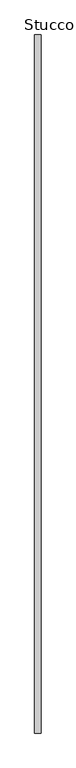
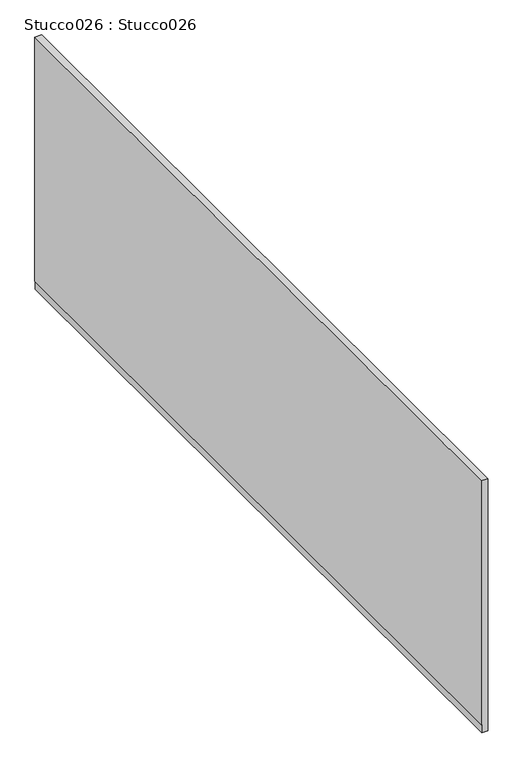
"""IFC4 building model written with IfcOpenShell, lengths in millimetres: proxy geometry, Stucco026 : Stucco026."""

from ifc_helpers import new_model, si_unit, frame, origin, place, context, project, spatial, polyline, outline, extrude, source, transform, mapped, element, save


def stucco026_stucco026_99b10f1b(model_context):
    return source(origin(), model_context, "Body", "SweptSolid", [
        extrude(outline(polyline([(39567.688258, -2790.7286469), (39567.688258, -2789.4428853), (39545.1576447, -2789.4428853), (39545.1576447, -2772.9484423), (40234.4061757, -2772.9484423), (40234.4061757, -2790.7286469), (39567.688258, -2790.7286469)])), frame((0.0, -1052.8905835, 0.0), z_axis=(0.0, 1.0, 0.0), x_axis=(0.0, 0.0, 1.0)), (0.0, 0.0, 1.0), 2000.0),
    ])


if __name__ == "__main__":
    model = new_model("IFC4")
    model_context = context("Model", 3, world=origin())
    ifc_project = project(units=[si_unit("LENGTHUNIT", "METRE", prefix="MILLI")], contexts=[model_context])
    site = spatial("IfcSite", under=ifc_project)
    building = spatial("IfcBuilding", under=site)
    placement = place(None, origin())
    stucco026_stucco026_shape = stucco026_stucco026_99b10f1b(model_context)
    element("IfcBuildingElementProxy", 1, Name="Stucco026 : Stucco026", ObjectType="Stucco026 : Stucco026", at=placement, inside=building, context=model_context, shape_type="MappedRepresentation", body=[
        mapped(stucco026_stucco026_shape, transform((0.0, 0.0, 0.0), x_axis=(1.0, 0.0, 0.0), y_axis=(0.0, 1.0, 0.0), z_axis=(0.0, 0.0, 1.0))),
    ])
    save(model, "model.ifc")

# Revit data of these elements
# Type "Stucco026 : Stucco026"
#   NameOverride = "Stucco026"
# Element 1 (IfcBuildingElementProxy, "Stucco026 : Stucco026")
#   Materials on its faces: "7/8\" SMOOTH TROWEL EXTERIOR STUCCO"
# Materials
#   "7/8\" SMOOTH TROWEL EXTERIOR STUCCO": class "Unassigned", colour RGB 255 255 255, transparency 0, Cost = 0
